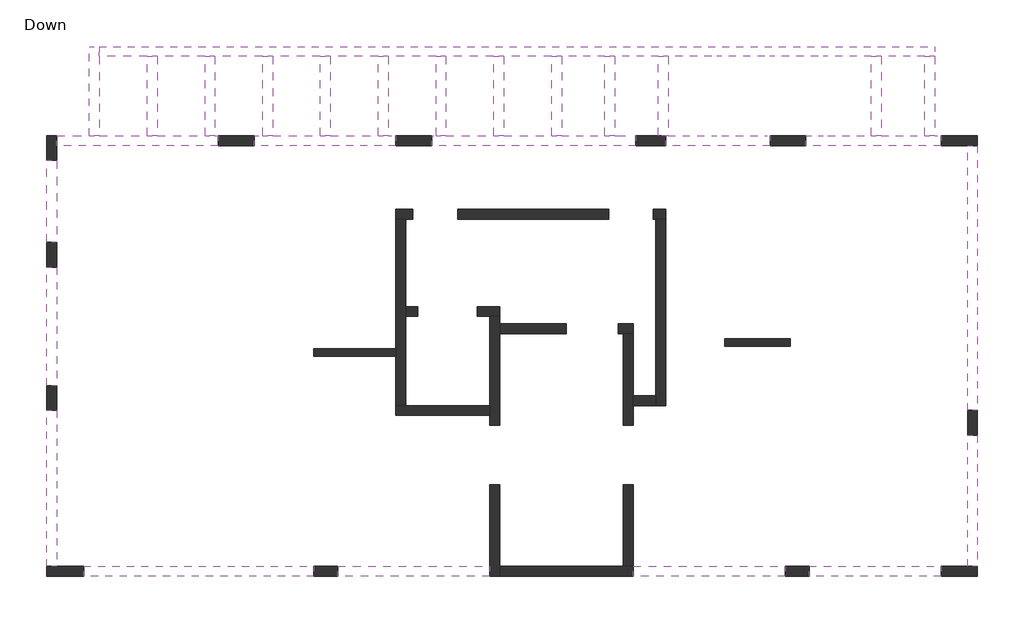
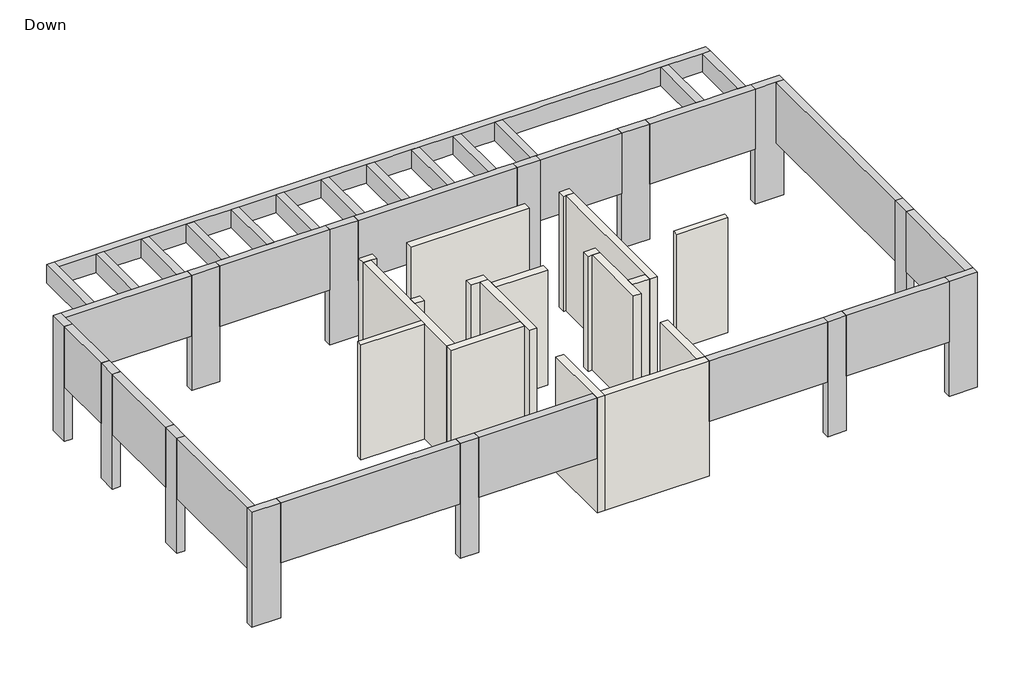
# One storey: 28 beams, 18 walls, 13 columns.
# Revit data of these elements (continued)
# Element 35 (IfcColumn, "Concrete Rectengular Column : 20/60") (continued)
#   Mark = "C7"
#   SOFiSTiK_AMG_Comments = ""
#   SOFiSTiK_AMG_Scheduled = yes
#   SOFiSTiK_AMG_Adjusted = yes
#   Structural Material = Concrete
#   Phase Created = New Construction
#   Materials on its faces: "Concrete"
# Element 36 (IfcColumn, "Concrete Rectengular Column : 20/72")
#   Comments = ""
#   Mark = "C8"
#   SOFiSTiK_AMG_Comments = ""
#   SOFiSTiK_AMG_Scheduled = yes
#   SOFiSTiK_AMG_Adjusted = yes
#   Structural Material = Concrete
#   Phase Created = New Construction
#   Materials on its faces: "Concrete"
# Element 37 (IfcColumn, "Concrete Rectengular Column : 20/73")
#   Comments = ""
#   Mark = "C9"
#   SOFiSTiK_AMG_Comments = ""
#   SOFiSTiK_AMG_Scheduled = yes
#   SOFiSTiK_AMG_Adjusted = yes
#   Structural Material = Concrete
#   Phase Created = New Construction
#   Materials on its faces: "Concrete"
# Element 38 (IfcColumn, "Concrete Rectengular Column : 20/73")
#   Comments = ""
#   Mark = "C10"
#   SOFiSTiK_AMG_Comments = ""
#   SOFiSTiK_AMG_Scheduled = yes
#   SOFiSTiK_AMG_Adjusted = yes
#   Structural Material = Concrete
#   Phase Created = New Construction
#   Materials on its faces: "Concrete"
# Element 39 (IfcColumn, "Concrete Rectengular Column : 20/73")
#   Comments = ""
#   Mark = "C11"
#   SOFiSTiK_AMG_Comments = ""
#   SOFiSTiK_AMG_Scheduled = yes
#   SOFiSTiK_AMG_Adjusted = yes
#   Structural Material = Concrete
#   Phase Created = New Construction
#   Materials on its faces: "Concrete"
# Element 40 (IfcColumn, "Concrete Rectengular Column : 20/73")
#   Comments = ""
#   Mark = "C12"
#   SOFiSTiK_AMG_Comments = ""
#   SOFiSTiK_AMG_Scheduled = yes
#   SOFiSTiK_AMG_Adjusted = yes
#   Structural Material = Concrete
#   Phase Created = New Construction
#   Materials on its faces: "Concrete"
# Element 41 (IfcColumn, "Concrete Rectengular Column : 20/75")
#   Comments = ""
#   Mark = "C13"
#   SOFiSTiK_AMG_Comments = ""
#   SOFiSTiK_AMG_Scheduled = yes
#   SOFiSTiK_AMG_Adjusted = yes
#   Structural Material = Concrete
#   Phase Created = New Construction
#   Materials on its faces: "Concrete"
# Element 42 (IfcWall, "15")
#   Comments = ""
#   Mark = "W18"
#   SOFiSTiK_AMG_Comments = ""
#   Top Offset = 0 cm
#   Base Offset = 0 cm
#   wall height = 315 cm
#   SOFiSTiK_AMG_Scheduled = yes
#   SOFiSTiK_AMG_Adjusted = yes
#   Phase Created = New Construction
#   Base Constraint = Down
#   Top Constraint = Typical Floor
#   Materials on its faces: "Concrete"
# Element 43 (IfcWall, "15")
#   Comments = ""
#   Mark = "W19"
#   SOFiSTiK_AMG_Comments = ""
#   Top Offset = 0 cm
#   Base Offset = 0 cm
#   wall height = 315 cm
#   SOFiSTiK_AMG_Scheduled = yes
#   SOFiSTiK_AMG_Adjusted = yes
#   Phase Created = New Construction
#   Base Constraint = Down
#   Top Constraint = Typical Floor
#   Materials on its faces: "Concrete"
# Element 44 (IfcWall, "20")
#   Comments = ""
#   Mark = "W1"
#   SOFiSTiK_AMG_Comments = ""
#   Top Offset = 0 cm
#   Base Offset = 0 cm
#   wall height = 315 cm
#   SOFiSTiK_AMG_Scheduled = yes
#   SOFiSTiK_AMG_Adjusted = yes
#   Phase Created = New Construction
#   Base Constraint = Down
#   Top Constraint = Typical Floor
#   Materials on its faces: "Concrete"
# Element 45 (IfcWall, "20")
#   Comments = ""
#   Mark = "W2"
#   SOFiSTiK_AMG_Comments = ""
#   Top Offset = 0 cm
#   Base Offset = 0 cm
#   wall height = 315 cm
#   SOFiSTiK_AMG_Scheduled = yes
#   SOFiSTiK_AMG_Adjusted = yes
#   Phase Created = New Construction
#   Base Constraint = Down
#   Top Constraint = Typical Floor
#   Materials on its faces: "Concrete"
# Element 46 (IfcWall, "20")
#   Comments = ""
#   Mark = "W3"
#   SOFiSTiK_AMG_Comments = ""
#   Top Offset = 0 cm
#   Base Offset = 0 cm
#   wall height = 315 cm
#   SOFiSTiK_AMG_Scheduled = yes
#   SOFiSTiK_AMG_Adjusted = yes
#   Phase Created = New Construction
#   Base Constraint = Down
#   Top Constraint = Typical Floor
#   Materials on its faces: "Concrete"
# Element 47 (IfcWall, "20")
#   Comments = ""
#   Mark = "W4"
#   SOFiSTiK_AMG_Comments = ""
#   Top Offset = 0 cm
#   Base Offset = 0 cm
#   wall height = 315 cm
#   SOFiSTiK_AMG_Scheduled = yes
#   SOFiSTiK_AMG_Adjusted = yes
#   Phase Created = New Construction
#   Base Constraint = Down
#   Top Constraint = Typical Floor
#   Materials on its faces: "Concrete"
# Element 48 (IfcWall, "20")
#   Comments = ""
#   Mark = "W5"
#   SOFiSTiK_AMG_Comments = ""
#   Top Offset = 0 cm
#   Base Offset = 0 cm
#   wall height = 315 cm
#   SOFiSTiK_AMG_Scheduled = yes
#   SOFiSTiK_AMG_Adjusted = yes
#   Phase Created = New Construction
#   Base Constraint = Down
#   Top Constraint = Typical Floor
#   Materials on its faces: "Concrete"
# Element 49 (IfcWall, "20")
#   Comments = ""
#   Mark = "W6"
#   SOFiSTiK_AMG_Comments = ""
#   Top Offset = 0 cm
#   Base Offset = 0 cm
#   wall height = 315 cm
#   SOFiSTiK_AMG_Scheduled = yes
#   SOFiSTiK_AMG_Adjusted = yes
#   Phase Created = New Construction
#   Base Constraint = Down
#   Top Constraint = Typical Floor
#   Materials on its faces: "Concrete"
# Element 50 (IfcWall, "20")
#   Comments = ""
#   Mark = "W7"
#   SOFiSTiK_AMG_Comments = ""
#   Top Offset = 0 cm
#   Base Offset = 0 cm
#   wall height = 315 cm
#   SOFiSTiK_AMG_Scheduled = yes
#   SOFiSTiK_AMG_Adjusted = yes
#   Phase Created = New Construction
#   Base Constraint = Down
#   Top Constraint = Typical Floor
#   Materials on its faces: "Concrete"
# Element 51 (IfcWall, "20")
#   Comments = ""
#   Mark = "W8"
#   SOFiSTiK_AMG_Comments = ""
#   Top Offset = 0 cm
#   Base Offset = 0 cm
#   wall height = 315 cm
#   SOFiSTiK_AMG_Scheduled = yes
#   SOFiSTiK_AMG_Adjusted = yes
#   Phase Created = New Construction
#   Base Constraint = Down
#   Top Constraint = Typical Floor
#   Materials on its faces: "Concrete"
# Element 52 (IfcWall, "20")
#   Comments = ""
#   Mark = "W9"
#   SOFiSTiK_AMG_Comments = ""
#   Top Offset = 0 cm
#   Base Offset = 0 cm
#   wall height = 315 cm
#   SOFiSTiK_AMG_Scheduled = yes
#   SOFiSTiK_AMG_Adjusted = yes
#   Phase Created = New Construction
#   Base Constraint = Down
#   Top Constraint = Typical Floor
#   Materials on its faces: "Concrete"
# Element 53 (IfcWall, "20")
#   Comments = ""
#   Mark = "W10"
#   SOFiSTiK_AMG_Comments = ""
#   Top Offset = 0 cm
#   Base Offset = 0 cm
#   wall height = 315 cm
#   SOFiSTiK_AMG_Scheduled = yes
#   SOFiSTiK_AMG_Adjusted = yes
#   Phase Created = New Construction
#   Base Constraint = Down
#   Top Constraint = Typical Floor
#   Materials on its faces: "Concrete"
# Element 54 (IfcWall, "20")
#   Comments = ""
#   Mark = "W11"
#   SOFiSTiK_AMG_Comments = ""
#   Top Offset = 0 cm
#   Base Offset = 0 cm
#   wall height = 315 cm
#   SOFiSTiK_AMG_Scheduled = yes
#   SOFiSTiK_AMG_Adjusted = yes
#   Phase Created = New Construction
#   Base Constraint = Down
#   Top Constraint = Typical Floor
#   Materials on its faces: "Concrete"
# Element 55 (IfcWall, "20")
#   Comments = ""
#   Mark = "W12"
#   SOFiSTiK_AMG_Comments = ""
#   Top Offset = 0 cm
#   Base Offset = 0 cm
#   wall height = 315 cm
#   SOFiSTiK_AMG_Scheduled = yes
#   SOFiSTiK_AMG_Adjusted = yes
#   Phase Created = New Construction
#   Base Constraint = Down
#   Top Constraint = Typical Floor
#   Materials on its faces: "Concrete"
# Element 56 (IfcWall, "20")
#   Comments = ""
#   Mark = "W13"
#   SOFiSTiK_AMG_Comments = ""
#   Top Offset = 0 cm
#   Base Offset = 0 cm
#   wall height = 315 cm
#   SOFiSTiK_AMG_Scheduled = yes
#   SOFiSTiK_AMG_Adjusted = yes
#   Phase Created = New Construction
#   Base Constraint = Down
#   Top Constraint = Typical Floor
#   Materials on its faces: "Concrete"
# Element 57 (IfcWall, "20")
#   Comments = ""
#   Mark = "W14"
#   SOFiSTiK_AMG_Comments = ""
#   Top Offset = 0 cm
#   Base Offset = 0 cm
#   wall height = 315 cm
#   SOFiSTiK_AMG_Scheduled = yes
#   SOFiSTiK_AMG_Adjusted = yes
#   Phase Created = New Construction
#   Base Constraint = Down
#   Top Constraint = Typical Floor
#   Materials on its faces: "Concrete"
# Element 58 (IfcWall, "20")
#   Comments = ""
#   Mark = "W16"
#   SOFiSTiK_AMG_Comments = ""
#   Top Offset = 0 cm
#   Base Offset = 0 cm
#   wall height = 315 cm
#   SOFiSTiK_AMG_Scheduled = yes
#   SOFiSTiK_AMG_Adjusted = yes
#   Phase Created = New Construction
#   Base Constraint = Down
#   Top Constraint = Typical Floor
#   Materials on its faces: "Concrete"
# Element 59 (IfcWall, "20")
#   Comments = ""
#   Mark = "W17"
#   SOFiSTiK_AMG_Comments = ""
#   Top Offset = 0 cm
#   Base Offset = 0 cm
#   wall height = 315 cm
#   SOFiSTiK_AMG_Scheduled = yes
#   SOFiSTiK_AMG_Adjusted = yes
#   Phase Created = New Construction
#   Base Constraint = Down
#   Top Constraint = Typical Floor
#   Materials on its faces: "Concrete"
# Materials
#   "Concrete": class "Concrete", colour RGB 192 192 192, transparency 0, Keynote = "01000", Description = "Cast-in-place concrete", Cost = 0
